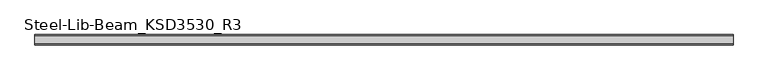
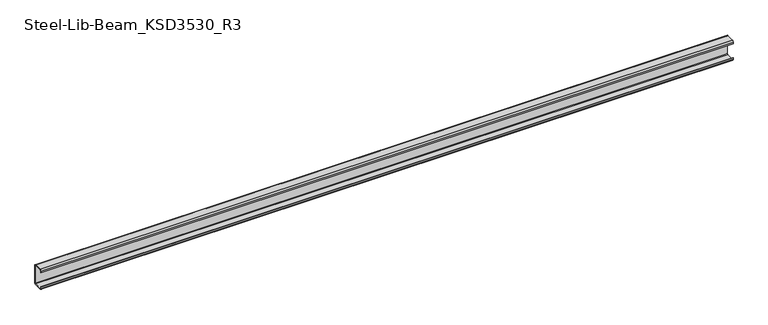
"""IFC4 building model written with IfcOpenShell, lengths in millimetres: beam geometry, Steel-Lib-Beam_KSD3530_R3 : BMS291_C-150×75x20x4.5."""

from ifc_helpers import new_model, si_unit, point, frame, frame_2d, origin, place, context, project, spatial, polyline, circle_curve, trimmed, segment, composite_curve, outline, extrude, source, transform, mapped, element, save


def steel_lib_beam_ksd3530_r3_1ba455c0(model_context):
    return source(origin(), model_context, "Body", "SweptSolid", [
        extrude(outline(composite_curve([segment(trimmed(circle_curve(frame_2d((-41.0, 66.0)), 9.0), [point((-50.0, 66.0))], [point((-41.0, 75.0))], False, "CARTESIAN"), True, "CONTINUOUS"), segment(polyline([(-41.0, 75.0), (16.0, 75.0)]), True, "CONTINUOUS"), segment(trimmed(circle_curve(frame_2d((16.0, 66.0)), 9.0), [point((16.0, 75.0))], [point((25.0, 66.0))], False, "CARTESIAN"), True, "CONTINUOUS"), segment(polyline([(25.0, 66.0), (25.0, -66.0)]), True, "CONTINUOUS"), segment(trimmed(circle_curve(frame_2d((16.0, -66.0)), 9.0), [point((25.0, -66.0))], [point((16.0, -75.0))], False, "CARTESIAN"), True, "CONTINUOUS"), segment(polyline([(16.0, -75.0), (-41.0, -75.0)]), True, "CONTINUOUS"), segment(trimmed(circle_curve(frame_2d((-41.0, -66.0)), 9.0), [point((-41.0, -75.0))], [point((-50.0, -66.0))], False, "CARTESIAN"), True, "CONTINUOUS"), segment(polyline([(-50.0, -66.0), (-50.0, -55.0), (-45.5, -55.0), (-45.5, -66.0)]), True, "CONTINUOUS"), segment(trimmed(circle_curve(frame_2d((-41.0, -66.0)), 4.5), [point((-45.5, -66.0))], [point((-41.0, -70.5))], True, "CARTESIAN"), True, "CONTINUOUS"), segment(polyline([(-41.0, -70.5), (16.0, -70.5)]), True, "CONTINUOUS"), segment(trimmed(circle_curve(frame_2d((16.0, -66.0)), 4.5), [point((16.0, -70.5))], [point((20.5, -66.0))], True, "CARTESIAN"), True, "CONTINUOUS"), segment(polyline([(20.5, -66.0), (20.5, 66.0)]), True, "CONTINUOUS"), segment(trimmed(circle_curve(frame_2d((16.0, 66.0)), 4.5), [point((20.5, 66.0))], [point((16.0, 70.5))], True, "CARTESIAN"), True, "CONTINUOUS"), segment(polyline([(16.0, 70.5), (-41.0, 70.5)]), True, "CONTINUOUS"), segment(trimmed(circle_curve(frame_2d((-41.0, 66.0)), 4.5), [point((-41.0, 70.5))], [point((-45.5, 66.0))], True, "CARTESIAN"), True, "CONTINUOUS"), segment(polyline([(-45.5, 66.0), (-45.5, 55.0), (-50.0, 55.0), (-50.0, 66.0)]), True, "CONTINUOUS")], self_intersect=False)), frame((-2490.0, 0.0, 0.0), z_axis=(1.0, 0.0, 0.0), x_axis=(0.0, 1.0, 0.0)), (0.0, 0.0, 1.0), 4980.0),
    ])


if __name__ == "__main__":
    model = new_model("IFC4")
    model_context = context("Model", 3, world=origin())
    ifc_project = project(units=[si_unit("LENGTHUNIT", "METRE", prefix="MILLI")], contexts=[model_context])
    site = spatial("IfcSite", under=ifc_project)
    building = spatial("IfcBuilding", under=site)
    placement = place(None, origin())
    steel_lib_beam_ksd3530_r3_shape = steel_lib_beam_ksd3530_r3_1ba455c0(model_context)
    element("IfcBeam", 1, ObjectType="Steel-Lib-Beam_KSD3530_R3 : BMS291_C-150×75x20x4.5", at=placement, inside=building, context=model_context, shape_type="MappedRepresentation", body=[
        mapped(steel_lib_beam_ksd3530_r3_shape, transform((0.0, 0.0, 0.0), x_axis=(1.0, 0.0, 0.0), y_axis=(0.0, 1.0, 0.0), z_axis=(0.0, 0.0, 1.0))),
    ])
    save(model, "model.ifc")

# Revit data of these elements
# Type "Steel-Lib-Beam_KSD3530_R3 : BMS291_C-150×75x20x4.5"
#   Keynote = "C-150×75x20x4.5"
#   SteelWeight = "Light"
#   x = 0.0250 m
#   t1 = 0.0090 m
#   t = 0.0045 m
#   Surface Area = 0.629834 m²/m
#   Section Area = 13.9688 cm²
#   Mass per Unit Length = 10.9655 kg/m
#   C = 0.0200 m
#   A = 0.0750 m
#   Length [instance default] = 1.5000 m
#   H = 0.1500 m
#   hec_material4 [instance default] = none
#   hec_material3 [instance default] = none
#   hec_material2 [instance default] = none
#   hec_material1 [instance default] = none
#   Structural Material [instance default] = Metal - Steel - Light Gauge
#   Assembly Code = ""
# Element 1 (IfcBeam, "Steel-Lib-Beam_KSD3530_R3 : BMS291_C-150×75x20x4.5")
#   Structural Material = none
# Materials
#   "Metal - Steel - Light Gauge": class "Metal", colour RGB 247 247 247, transparency 0
